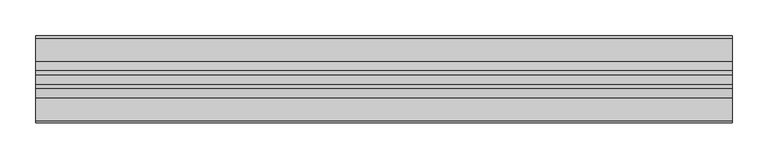
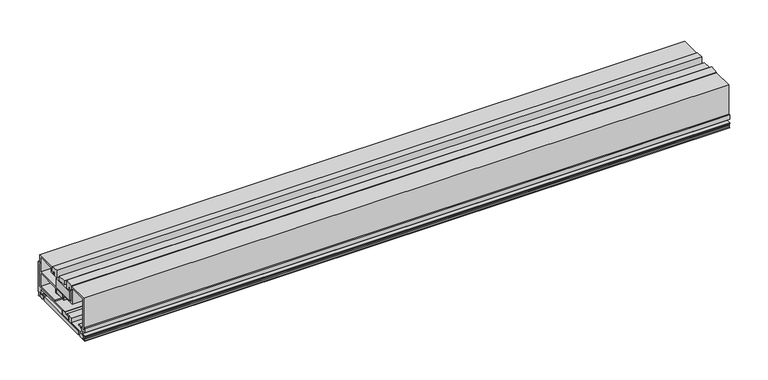
"""IFC4 building model written with IfcOpenShell, lengths in millimetres: proxy geometry, Generic Models 3:Generic Models 1:2:Generic Models 1:2 : Generic Models 3:Generic Models 1:300625:328150:Generic Models 1:2:Generic Models 1:2 : Generic Models 3:Generic Models 1:300625:328150 : Generic Models 3:Generic Models 1:2:Generic Models 1:2 : Generic Models 3:Generic Models 1:300625:328150:6 : Generic Models 3:Generic Models 1:2:Generic Models 1:2 : Generic Models 3:Generic Models 1:300625:328150:Generic Models 1:2:Generic Models 1:2 : Generic Models 3:Generic Models 1:300625:328150 : Generic Models 3:Generic Models 1:2:Generic Models 1:2 : Generic Models 3:Generic Models 1:300625:328150:300962."""

from ifc_helpers import new_model, si_unit, frame, origin, origin_with_axes, place, context, project, spatial, polyline, outline, extrude, source, transform, mapped, element, save


def generic_models_b114195a(model_context):
    return source(origin(), model_context, "Body", "SweptSolid", [
        extrude(outline(polyline([(593657.1242239, -579015.3141007), (593657.1242239, -579104.2141007), (592761.7742239, -579104.2141007), (592761.7742239, -579015.3141007), (593657.1242239, -579015.3141007)])), origin_with_axes(), (0.0, 0.0, 1.0), 6.35),
        extrude(outline(polyline([(-579000.519923, 5.3842368), (-579000.8336091, 3.175), (-579000.519923, 0.9657632), (-579000.1425144, 0.0), (-579006.0106065, 0.0), (-579005.1503256, 0.3863176), (-579003.8407504, 1.469803), (-579003.2403969, 2.8200508), (-579003.4431848, 4.2258271), (-579004.4173898, 5.4672112), (-579006.0106065, 6.35), (-579000.1425144, 6.35), (-579000.519923, 5.3842368)])), frame((592761.7742239, 0.0, 0.0), z_axis=(1.0, 0.0, 0.0), x_axis=(0.0, 1.0, 0.0)), (0.0, 0.0, 1.0), 895.35),
        extrude(outline(polyline([(-579004.0833699, 1.7974191), (-579005.4048639, 0.692685), (-579007.3144782, 0.0796039), (-579008.3742341, 0.0), (-579009.4339901, 0.0796039), (-579011.3436043, 0.692685), (-579012.6650983, 1.7974191), (-579013.1367341, 3.175), (-579012.6650983, 4.5525809), (-579011.3436043, 5.657315), (-579009.4339901, 6.2703961), (-579008.3742341, 6.35), (-579007.3144782, 6.2703961), (-579005.4048639, 5.657315), (-579004.0833699, 4.5525809), (-579003.6117341, 3.175), (-579004.0833699, 1.7974191)])), frame((592761.7742239, 0.0, 0.0), z_axis=(1.0, 0.0, 0.0), x_axis=(0.0, 1.0, 0.0)), (0.0, 0.0, 1.0), 895.35),
        extrude(outline(polyline([(-579111.68681, 0.0796039), (-579112.746566, 0.0), (-579113.8063219, 0.0796039), (-579115.7159362, 0.692685), (-579117.0374302, 1.7974191), (-579117.509066, 3.175), (-579117.0374302, 4.5525809), (-579115.7159362, 5.657315), (-579113.8063219, 6.2703961), (-579112.746566, 6.35), (-579111.68681, 6.2703961), (-579109.7771958, 5.657315), (-579108.4557018, 4.5525809), (-579107.984066, 3.175), (-579108.4557018, 1.7974191), (-579109.7771958, 0.692685), (-579111.68681, 0.0796039)])), frame((592761.7742239, 0.0, 0.0), z_axis=(1.0, 0.0, 0.0), x_axis=(0.0, 1.0, 0.0)), (0.0, 0.0, 1.0), 969.9625),
        extrude(outline(polyline([(-579115.1101936, 0.0), (-579120.9782857, 0.0), (-579120.6008771, 0.9657632), (-579120.287191, 3.175), (-579120.6008771, 5.3842368), (-579120.9782857, 6.35), (-579115.1101936, 6.35), (-579116.7034103, 5.4672112), (-579117.6776153, 4.2258271), (-579117.8804032, 2.8200508), (-579117.2800497, 1.469803), (-579115.9704745, 0.3863176), (-579115.1101936, 0.0)])), frame((592761.7742239, 0.0, 0.0), z_axis=(1.0, 0.0, 0.0), x_axis=(0.0, 1.0, 0.0)), (0.0, 0.0, 1.0), 969.9625),
        extrude(outline(polyline([(593731.7367239, -579047.2017564), (593731.7367239, -579080.4885915), (592761.7742239, -579080.4885915), (592761.7742239, -579047.2017564), (593731.7367239, -579047.2017564)])), frame((0.0, 0.0, 40.9290939), z_axis=(0.0, 0.0, 1.0), x_axis=(1.0, 0.0, 0.0)), (0.0, 0.0, 1.0), 14.2115027),
        extrude(outline(polyline([(593731.7367239, -579063.676291), (593731.7367239, -579079.7877272), (592761.7742239, -579079.7877272), (592761.7742239, -579063.676291), (593731.7367239, -579063.676291)])), frame((0.0, 0.0, 8.0979388), z_axis=(0.0, 0.0, 1.0), x_axis=(1.0, 0.0, 0.0)), (0.0, 0.0, 1.0), 6.0797872),
        extrude(outline(polyline([(-579003.1775737, 53.9246391), (-579000.1425144, 53.9246391), (-579000.1425144, 6.35), (-579008.035108, 6.35), (-579008.035108, 13.721742), (-579062.0043495, 13.721742), (-579062.0043495, 6.35), (-579068.5401208, 6.35), (-579068.5401208, 8.0979388), (-579063.676291, 8.0979388), (-579063.676291, 14.1777261), (-579068.5401208, 14.1777261), (-579068.5401208, 15.4696809), (-579001.8904532, 15.4696809), (-579001.8904532, 52.2575319), (-579003.1775737, 52.2575319), (-579003.1775737, 53.9246391)])), frame((592761.7742239, 0.0, 0.0), z_axis=(1.0, 0.0, 0.0), x_axis=(0.0, 1.0, 0.0)), (0.0, 0.0, 1.0), 969.9625),
        extrude(outline(polyline([(-579085.6315392, 8.0979388), (-579085.6315392, 15.4696809), (-579074.9238974, 15.4696809), (-579074.9238974, 14.1777261), (-579079.7877272, 14.1777261), (-579079.7877272, 8.0979388), (-579074.9238974, 8.0979388), (-579074.9238974, 6.35), (-579120.9782857, 6.35), (-579120.9782857, 8.0979388), (-579114.5945091, 8.0979388), (-579114.5945091, 13.721742), (-579120.9782857, 13.721742), (-579120.9782857, 20.2285817), (-579119.1114916, 20.2285817), (-579119.1114916, 15.4696809), (-579110.1654191, 15.4696809), (-579110.1654191, 14.5730392), (-579112.5861229, 13.9244136), (-579111.6757362, 8.0979388), (-579085.6315392, 8.0979388)])), frame((592761.7742239, 0.0, 0.0), z_axis=(1.0, 0.0, 0.0), x_axis=(0.0, 1.0, 0.0)), (0.0, 0.0, 1.0), 969.9625),
        extrude(outline(polyline([(593731.7367239, -579047.8857325), (593731.7367239, -579063.9971687), (592761.7742239, -579063.9971687), (592761.7742239, -579047.8857325), (593731.7367239, -579047.8857325)])), frame((0.0, 0.0, 32.9493731), z_axis=(0.0, 0.0, 1.0), x_axis=(1.0, 0.0, 0.0)), (0.0, 0.0, 1.0), 6.0797872),
        extrude(outline(polyline([(593731.7367239, -579054.6832724), (593731.7367239, -579067.3832724), (592761.7742239, -579067.3832724), (592761.7742239, -579054.6832724), (593731.7367239, -579054.6832724)])), frame((0.0, 0.0, 57.1165274), z_axis=(0.0, 0.0, 1.0), x_axis=(1.0, 0.0, 0.0)), (0.0, 0.0, 1.0), 6.3435484),
        extrude(outline(polyline([(-579078.8757591, 62.433193), (-579081.7214373, 62.433193), (-579081.7214373, 59.4893332), (-579086.0195091, 59.4893332), (-579086.0195091, 67.3290426), (-579074.1217032, 68.7899095), (-579074.1217032, 56.7196524), (-579078.8757591, 56.7196524), (-579078.8757591, 62.433193)])), frame((592761.7742239, 0.0, 0.0), z_axis=(1.0, 0.0, 0.0), x_axis=(0.0, 1.0, 0.0)), (0.0, 0.0, 1.0), 969.9625),
        extrude(outline(polyline([(-579036.0470357, 67.3290426), (-579036.0470357, 59.4893332), (-579040.3451075, 59.4893332), (-579040.3451075, 62.433193), (-579043.1907857, 62.433193), (-579043.1907857, 56.7196524), (-579047.9448415, 56.7196524), (-579047.9448415, 68.7899095), (-579036.0470357, 67.3290426)])), frame((592761.7742239, 0.0, 0.0), z_axis=(1.0, 0.0, 0.0), x_axis=(0.0, 1.0, 0.0)), (0.0, 0.0, 1.0), 969.9625),
        extrude(outline(polyline([(-579118.1663841, 15.5459822), (-579118.1663841, 66.3122056), (-579086.4163841, 66.3122056), (-579086.4163841, 59.0924582), (-579081.3245623, 59.0924582), (-579081.3245623, 62.036318), (-579079.2726341, 62.036318), (-579079.2726341, 57.1165274), (-579086.4163841, 57.1165274), (-579086.4163841, 40.9290939), (-579059.1333389, 40.9290939), (-579059.1333389, 39.0291604), (-579063.9971687, 39.0291604), (-579063.9971687, 32.9493731), (-579059.1333389, 32.9493731), (-579059.1333389, 31.6574183), (-579065.8971022, 31.6574183), (-579065.8971022, 39.0291604), (-579088.3163176, 39.0291604), (-579088.3163176, 64.4122721), (-579115.6584719, 64.4122721), (-579115.6584719, 17.4459157), (-579105.079253, 17.4459157), (-579105.079253, 15.5459822), (-579118.1663841, 15.5459822)])), frame((592761.7742239, 0.0, 0.0), z_axis=(1.0, 0.0, 0.0), x_axis=(0.0, 1.0, 0.0)), (0.0, 0.0, 1.0), 969.9625),
        extrude(outline(polyline([(-579040.7419825, 62.036318), (-579040.7419825, 59.0924582), (-579035.6501607, 59.0924582), (-579035.6501607, 66.3122056), (-579003.8663841, 66.3122056), (-579003.8663841, 15.5459822), (-579042.7939107, 15.5459822), (-579042.7939107, 17.4681948), (-579005.8423149, 17.4681948), (-579005.8423149, 39.0291604), (-579045.985799, 39.0291604), (-579045.985799, 31.6574183), (-579052.7495623, 31.6574183), (-579052.7495623, 32.9493731), (-579047.8857325, 32.9493731), (-579047.8857325, 39.0291604), (-579052.7495623, 39.0291604), (-579052.7495623, 40.9290939), (-579005.8423149, 40.9290939), (-579005.8423149, 64.4024065), (-579033.7502272, 64.4024065), (-579033.7502272, 57.1165274), (-579042.7939107, 57.1165274), (-579042.7939107, 62.036318), (-579040.7419825, 62.036318)])), frame((592761.7742239, 0.0, 0.0), z_axis=(1.0, 0.0, 0.0), x_axis=(0.0, 1.0, 0.0)), (0.0, 0.0, 1.0), 969.9625),
    ])


if __name__ == "__main__":
    model = new_model("IFC4")
    model_context = context("Model", 3, world=origin())
    ifc_project = project(units=[si_unit("LENGTHUNIT", "METRE", prefix="MILLI")], contexts=[model_context])
    site = spatial("IfcSite", under=ifc_project)
    building = spatial("IfcBuilding", under=site)
    placement = place(None, origin())
    generic_models_shape = generic_models_b114195a(model_context)
    element("IfcBuildingElementProxy", 1, Name="Generic Models 3:Generic Models 1:2:Generic Models 1:2 : Generic Models 3:Generic Models 1:300625:328150:Generic Models 1:2:Generic Models 1:2 : Generic Models 3:Generic Models 1:300625:328150 : Generic Models 3:Generic Models 1:2:Generic Models 1:2 : Generic Models 3:Generic Models 1:300625:328150:6 : Generic Models 3:Generic Models 1:2:Generic Models 1:2 : Generic Models 3:Generic Models 1:300625:328150:Generic Models 1:2:Generic Models 1:2 : Generic Models 3:Generic Models 1:300625:328150 : Generic Models 3:Generic Models 1:2:Generic Models 1:2 : Generic Models 3:Generic Models 1:300625:328150:300962", ObjectType="Generic Models 3:Generic Models 1:2:Generic Models 1:2 : Generic Models 3:Generic Models 1:300625:328150:Generic Models 1:2:Generic Models 1:2 : Generic Models 3:Generic Models 1:300625:328150 : Generic Models 3:Generic Models 1:2:Generic Models 1:2 : Generic Models 3:Generic Models 1:300625:328150:6 : Generic Models 3:Generic Models 1:2:Generic Models 1:2 : Generic Models 3:Generic Models 1:300625:328150:Generic Models 1:2:Generic Models 1:2 : Generic Models 3:Generic Models 1:300625:328150 : Generic Models 3:Generic Models 1:2:Generic Models 1:2 : Generic Models 3:Generic Models 1:300625:328150:300962", at=placement, inside=building, context=model_context, shape_type="MappedRepresentation", body=[
        mapped(generic_models_shape, transform((0.0, 0.0, 0.0), x_axis=(1.0, 0.0, 0.0), y_axis=(0.0, 1.0, 0.0), z_axis=(0.0, 0.0, 1.0))),
    ])
    save(model, "model.ifc")

# Revit data of these elements
# Type "Generic Models 3:Generic Models 1:2:Generic Models 1:2 : Generic Models 3:Generic Models 1:300625:328150:Generic Models 1:2:Generic Models 1:2 : Generic Models 3:Generic Models 1:300625:328150 : Generic Models 3:Generic Models 1:2:Generic Models 1:2 : Generic Models 3:Generic Models 1:300625:328150:6 : Generic Models 3:Generic Models 1:2:Generic Models 1:2 : Generic Models 3:Generic Models 1:300625:328150:Generic Models 1:2:Generic Models 1:2 : Generic Models 3:Generic Models 1:300625:328150 : Generic Models 3:Generic Models 1:2:Generic Models 1:2 : Generic Models 3:Generic Models 1:300625:328150:300962"
#   NameOverride = "Generic Models 3:Generic Models 1:2:Generic Models 1:2 : Generic Models 3:Generic Models 1:300625:328150:Generic Models 1:2:Generic Models 1:2 : Generic Models 3:Generic Models 1:300625:328150 : Generic Models 3:Generic Models 1:2:Generic Models 1:2 : Generic Models 3:Generic Models 1:300625:328150:300962"
#   ObjectTypeOverride = "Generic Models 1:2:Generic Models 1:2 : Generic Models 3:Generic Models 1:300625:328150 : Generic Models 3:Generic Models 1:2:Generic Models 1:2 : Generic Models 3:Generic Models 1:300625:328150"
#   Reference = "Generic Models 1"
#   Tag = "300962"
# Element 1 (IfcBuildingElementProxy, "Generic Models 3:Generic Models 1:2:Generic Models 1:2 : Generic Models 3:Generic Models 1:300625:328150:Generic Models 1:2:Generic Models 1:2 : Generic Models 3:Generic Models 1:300625:328150 : Generic Models 3:Generic Models 1:2:Generic Models 1:2 : Generic Models 3:Generic Models 1:300625:328150:6 : Generic Models 3:Generic Models 1:2:Generic Models 1:2 : Generic Models 3:Generic Models 1:300625:328150:Generic Models 1:2:Generic Models 1:2 : Generic Models 3:Generic Models 1:300625:328150 : Generic Models 3:Generic Models 1:2:Generic Models 1:2 : Generic Models 3:Generic Models 1:300625:328150:300962")
#   Materials on its faces: "THERMAL BROKEN ALUMINUM STOREFRONT", "SEALANT & BACKER ROD", "Compression Gasket_1", "Shim_1", "Desiccant Sealant_1"
# Materials
#   "THERMAL BROKEN ALUMINUM STOREFRONT": class "Unassigned", colour RGB 244 244 244, transparency 0, Cost = 0
#   "SEALANT & BACKER ROD": class "Unassigned", colour RGB 120 120 120, transparency 0, Cost = 0
#   "Compression Gasket_1": class "Unassigned", colour RGB 178 178 178, transparency 0
#   "Shim_1": class "Unassigned", colour RGB 218 218 218, transparency 0
#   "Desiccant Sealant_1": class "Unassigned", colour RGB 120 120 120, transparency 0
